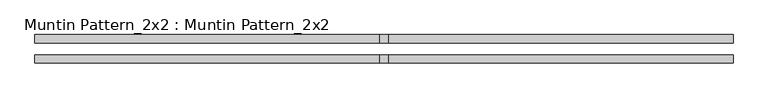
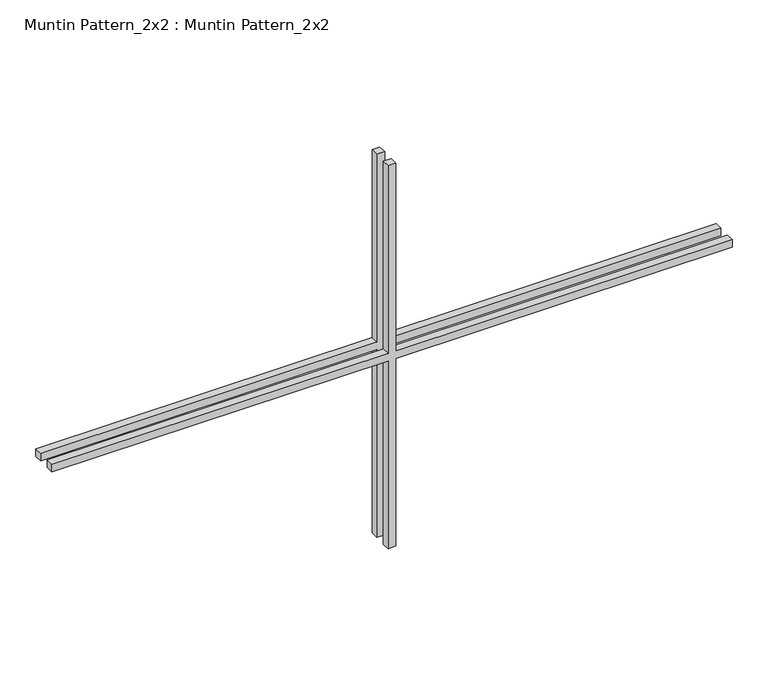
"""IFC4 building model written with IfcOpenShell, lengths in millimetres: proxy geometry, Muntin Pattern_2x2 : Muntin Pattern_2x2."""

import ifcopenshell
import ifcopenshell.guid

model = None  # the IFC model being written
_history = None  # IfcOwnerHistory: only IFC2X3 demands one
_inside = {}  # id of a spatial element -> (the spatial element, [elements in it])
_under = {}  # id of a project, library or spatial element -> (it, [spatial elements below it])
_declared = {}  # id of a project -> (the project, [libraries it declares])
_typed = {}  # id of a type object -> (the type object, [elements of that type])
_made_of = {}  # id of a material, layer set ... -> (it, [elements and type objects made of it])


def new_model(schema):
    """Start an empty IFC model of exactly this schema.

    Asked for "IFC4X3", IfcOpenShell would pick the latest addendum, in which some entities
    have other attributes; the version numbers below select the first issue.
    IFC2X3 requires an IfcOwnerHistory on every rooted entity: one is made here for all.
    """
    global model, _history
    if schema == "IFC4X3":
        model = ifcopenshell.file(schema_version=(4, 3, 0, 0))
    else:
        model = ifcopenshell.file(schema=schema)
    _inside.clear()
    _under.clear()
    _declared.clear()
    _typed.clear()
    _made_of.clear()
    _history = None
    if model.schema == "IFC2X3":
        org = make("IfcOrganization", Name="unknown")
        user = make(
            "IfcPersonAndOrganization",
            ThePerson=make("IfcPerson", FamilyName="unknown"),
            TheOrganization=org,
        )
        app = make(
            "IfcApplication",
            ApplicationDeveloper=org,
            Version="unknown",
            ApplicationFullName="unknown",
            ApplicationIdentifier="unknown",
        )
        _history = make(
            "IfcOwnerHistory",
            OwningUser=user,
            OwningApplication=app,
            ChangeAction="ADDED",
            CreationDate=0,
        )
    return model


def make(cls, **values):
    """One entity of the class cls with the attributes given. An attribute that is None is left unset."""
    return model.create_entity(
        cls, **{name: value for name, value in values.items() if value is not None}
    )


def rooted(cls, **values):
    """An entity with a GlobalId (a new one), such as an element, a storey or a relation."""
    return make(cls, GlobalId=ifcopenshell.guid.new(), OwnerHistory=_history, **values)


def si_unit(unit_type, name, prefix=None):
    """IfcSIUnit, for example si_unit("LENGTHUNIT", "METRE", prefix="MILLI")."""
    return make("IfcSIUnit", UnitType=unit_type, Prefix=prefix, Name=name)


def assignment(units):
    """IfcUnitAssignment: the units of a project."""
    return None if units is None else make("IfcUnitAssignment", Units=units)


def point(xyz):
    """IfcCartesianPoint."""
    return None if xyz is None else make("IfcCartesianPoint", Coordinates=xyz)


def direction(xyz):
    """IfcDirection."""
    return None if xyz is None else make("IfcDirection", DirectionRatios=xyz)


def frame(location, z_axis=None, x_axis=None):
    """IfcAxis2Placement3D, a coordinate frame: its origin and axes. An axis left out is left unset."""
    return make(
        "IfcAxis2Placement3D",
        Location=point(location),
        Axis=direction(z_axis),
        RefDirection=direction(x_axis),
    )


def origin():
    """The frame at (0, 0, 0) with its axes left unset."""
    return frame((0.0, 0.0, 0.0))


def place(relative_to, where):
    """IfcLocalPlacement: puts the frame where relative to a parent placement (None: the world)."""
    return make(
        "IfcLocalPlacement", PlacementRelTo=relative_to, RelativePlacement=where
    )


def context(
    kind, dimensions, precision=None, world=None, true_north=None, identifier=None
):
    """IfcGeometricRepresentationContext, for example the 3D "Model" context."""
    return make(
        "IfcGeometricRepresentationContext",
        ContextIdentifier=identifier,
        ContextType=kind,
        CoordinateSpaceDimension=dimensions,
        Precision=precision,
        WorldCoordinateSystem=world,
        TrueNorth=true_north,
    )


def project(units=None, contexts=None):
    """IfcProject with its units and contexts."""
    return rooted(
        "IfcProject",
        Name="project",
        RepresentationContexts=contexts,
        UnitsInContext=assignment(units),
    )


def spatial(cls, under=None, at=None, **own):
    """A site, building, storey or space (cls), placed at a placement, below another one or the project."""
    s = rooted(cls, ObjectPlacement=at, **own)
    if under is not None:
        _under.setdefault(under.id(), (under, []))[1].append(s)
    return s


def polyline(points):
    """IfcPolyline through the points."""
    return make("IfcPolyline", Points=[point(p) for p in points])


def outline(outer, holes=None, kind="AREA"):
    """IfcArbitraryClosedProfileDef: a profile drawn as a closed curve; with holes, ...WithVoids."""
    if holes is None:
        return make("IfcArbitraryClosedProfileDef", ProfileType=kind, OuterCurve=outer)
    return make(
        "IfcArbitraryProfileDefWithVoids",
        ProfileType=kind,
        OuterCurve=outer,
        InnerCurves=holes,
    )


def extrude(swept, where, along, depth):
    """IfcExtrudedAreaSolid: the profile swept, set in the frame where, extruded along a direction by depth."""
    return make(
        "IfcExtrudedAreaSolid",
        SweptArea=swept,
        Position=where,
        ExtrudedDirection=direction(along),
        Depth=depth,
    )


def shape(context_of_items, identifier, shape_type, items):
    """IfcShapeRepresentation: the items that make up one representation, for example the "Body"."""
    return make(
        "IfcShapeRepresentation",
        ContextOfItems=context_of_items,
        RepresentationIdentifier=identifier,
        RepresentationType=shape_type,
        Items=items,
    )


def source(mapping_origin, context_of_items, identifier, shape_type, items):
    """IfcRepresentationMap: a shape defined once, which mapped items show again and again."""
    return make(
        "IfcRepresentationMap",
        MappingOrigin=mapping_origin,
        MappedRepresentation=shape(context_of_items, identifier, shape_type, items),
    )


def transform(
    local_origin,
    x_axis=None,
    y_axis=None,
    z_axis=None,
    scale=None,
    scale2=None,
    scale3=None,
    uniform=True,
):
    """IfcCartesianTransformationOperator3D, or its non-uniform kind. x_axis, y_axis, z_axis: its Axis1, 2, 3."""
    if uniform:
        return make(
            "IfcCartesianTransformationOperator3D",
            Axis1=direction(x_axis),
            Axis2=direction(y_axis),
            LocalOrigin=point(local_origin),
            Scale=scale,
            Axis3=direction(z_axis),
        )
    return make(
        "IfcCartesianTransformationOperator3DnonUniform",
        Axis1=direction(x_axis),
        Axis2=direction(y_axis),
        LocalOrigin=point(local_origin),
        Scale=scale,
        Axis3=direction(z_axis),
        Scale2=scale2,
        Scale3=scale3,
    )


def mapped(mapping_source, mapping_target):
    """IfcMappedItem: shows the shape of a source again, moved by a transform."""
    return make(
        "IfcMappedItem", MappingSource=mapping_source, MappingTarget=mapping_target
    )


def made_of(thing, what):
    """Note that an element or type object is made of a material, layer set ...; save() writes the relation."""
    if what is not None:
        _made_of.setdefault(what.id(), (what, []))[1].append(thing)
    return thing


def element(
    cls,
    number,
    at=None,
    inside=None,
    cuts=None,
    type_object=None,
    material=None,
    context=None,
    identifier="Body",
    shape_type=None,
    held_by="IfcProductDefinitionShape",
    body=None,
    shapes=None,
    **own,
):
    """One element of the class cls, such as IfcWall. Its Tag is "e" and its number.

    at: its placement. inside: the storey or other place that contains it. cuts: it is an
    opening in that element (IfcRelVoidsElement). A single representation is given by context,
    identifier, shape_type and body (its items); several are given by shapes. held_by: the class
    of the entity that holds the representations. save() writes the other relations.
    """
    e = rooted(cls, Tag="e%d" % number, ObjectPlacement=at, **own)
    if body is not None:
        shapes = [shape(context, identifier, shape_type, body)]
    if shapes is not None:
        e.Representation = make(held_by, Representations=shapes)
    if inside is not None:
        _inside.setdefault(inside.id(), (inside, []))[1].append(e)
    if cuts is not None:
        rooted(
            "IfcRelVoidsElement", RelatingBuildingElement=cuts, RelatedOpeningElement=e
        )
    if type_object is not None:
        _typed.setdefault(type_object.id(), (type_object, []))[1].append(e)
    return made_of(e, material)


def aggregate(whole, parts):
    """IfcRelAggregates: a whole, such as a stair, and the parts it consists of."""
    return rooted("IfcRelAggregates", RelatingObject=whole, RelatedObjects=parts)


def save(model, path):
    """Write the relations noted so far, then the file.

    IfcRelAggregates (storeys below a building ...), IfcRelContainedInSpatialStructure (elements
    in a storey), IfcRelDefinesByType, IfcRelAssociatesMaterial and IfcRelDeclares: one each for
    every whole, place, type object, material and project.
    """
    for whole, parts in _under.values():
        aggregate(whole, parts)
    for where, things in _inside.values():
        rooted(
            "IfcRelContainedInSpatialStructure",
            RelatedElements=things,
            RelatingStructure=where,
        )
    for kind, things in _typed.values():
        rooted("IfcRelDefinesByType", RelatedObjects=things, RelatingType=kind)
    for what, things in _made_of.values():
        rooted("IfcRelAssociatesMaterial", RelatedObjects=things, RelatingMaterial=what)
    for by, libraries in _declared.values():
        rooted("IfcRelDeclares", RelatingContext=by, RelatedDefinitions=libraries)
    model.write(path)


def muntin_pattern_2x2_muntin_pattern_2x2_2b08dfa8(model_context):
    return source(origin(), model_context, "Body", "SweptSolid", [
        extrude(outline(polyline([(331.7875, -6.35), (331.7875, -546.1), (319.0875, -546.1), (319.0875, -6.35), (0.0, -6.35), (0.0, 6.35), (319.0875, 6.35), (319.0875, 546.1), (331.7875, 546.1), (331.7875, 6.35), (650.875, 6.35), (650.875, -6.35), (331.7875, -6.35)])), frame((0.0, 9.525, 0.0), z_axis=(0.0, 1.0, 0.0), x_axis=(0.0, 0.0, 1.0)), (0.0, 0.0, 1.0), 12.7),
        extrude(outline(polyline([(331.7875, -6.35), (331.7875, -546.1), (319.0875, -546.1), (319.0875, -6.35), (0.0, -6.35), (0.0, 6.35), (319.0875, 6.35), (319.0875, 546.1), (331.7875, 546.1), (331.7875, 6.35), (650.875, 6.35), (650.875, -6.35), (331.7875, -6.35)])), frame((0.0, -22.225, 0.0), z_axis=(0.0, 1.0, 0.0), x_axis=(0.0, 0.0, 1.0)), (0.0, 0.0, 1.0), 12.7),
    ])


if __name__ == "__main__":
    model = new_model("IFC4")
    model_context = context("Model", 3, world=origin())
    ifc_project = project(units=[si_unit("LENGTHUNIT", "METRE", prefix="MILLI")], contexts=[model_context])
    site = spatial("IfcSite", under=ifc_project)
    building = spatial("IfcBuilding", under=site)
    placement = place(None, origin())
    muntin_pattern_2x2_muntin_pattern_2x2_shape = muntin_pattern_2x2_muntin_pattern_2x2_2b08dfa8(model_context)
    element("IfcBuildingElementProxy", 1, Name="Muntin Pattern_2x2 : Muntin Pattern_2x2", ObjectType="Muntin Pattern_2x2 : Muntin Pattern_2x2", at=placement, inside=building, context=model_context, shape_type="MappedRepresentation", body=[
        mapped(muntin_pattern_2x2_muntin_pattern_2x2_shape, transform((0.0, 0.0, 0.0), x_axis=(1.0, 0.0, 0.0), y_axis=(0.0, 1.0, 0.0), z_axis=(0.0, 0.0, 1.0))),
    ])
    save(model, "model.ifc")

# Revit data of these elements
# Type "Muntin Pattern_2x2 : Muntin Pattern_2x2"
#   Width [instance default] = 4' - 0"
#   Thickness = 0' - 0 1/2"
#   Height [instance default] = 4' - 0"
#   Distance = 0' - 0 3/4"
#   Interior Material [instance default] = none
#   Exterior Material [instance default] = none
# Element 1 (IfcBuildingElementProxy, "Muntin Pattern_2x2 : Muntin Pattern_2x2")
#   Width = 3' - 7"
#   Height = 2' - 1 5/8"
#   Interior Material = Wood - Stained
#   Exterior Material = Clad - White
#   Materials on its faces: "Clad - White", "Wood - Stained"
# Materials
#   "Clad - White": class "Wood", colour RGB 242 242 238, transparency 0, Cost = 0
#   "Wood - Stained": class "Wood", colour RGB 224 178 126, transparency 0, Cost = 0
